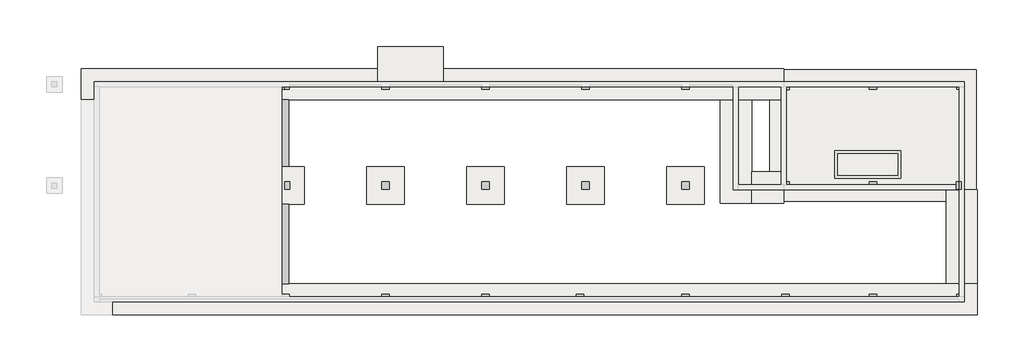
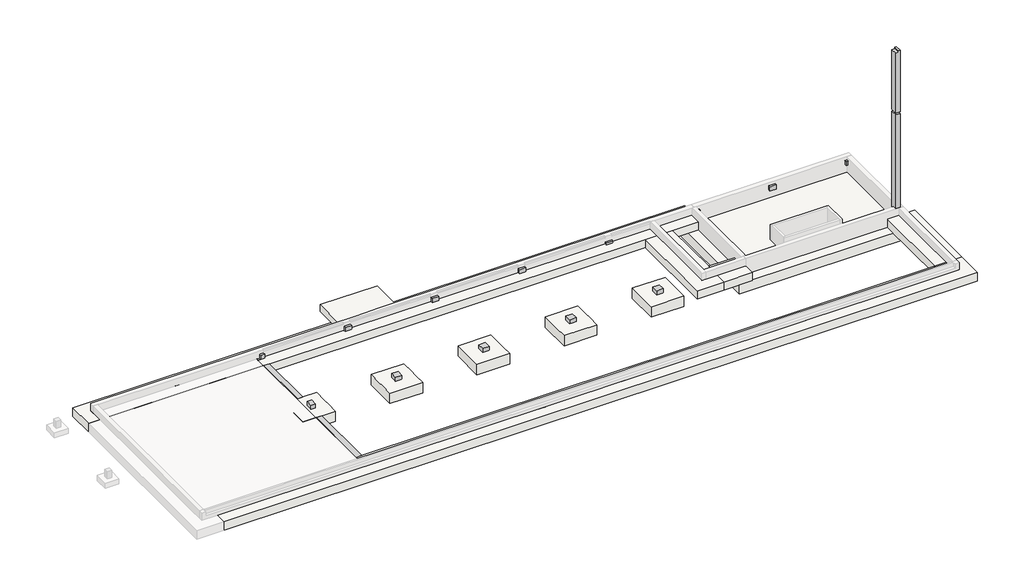
# Not in any storey, part 2 of 2: 25 columns, 8 beams, 8 slabs, 5 footings.
# Revit data of these elements (continued)
# Type "H_SF_AR_B01_MAT_Bitumen_MF2" (continued)
#   H_WM Code_3 = "A03AF036-00001 |  | M2 | Concrete Work | Superstructure Work | Form Work (1 time in use) | Flat Form | Dressed Lumber, Plywood or Steel Form(Wood Planks are not Allowed) incl. Chamfer |  |  |  | A03AF036-00001 Concrete Work Superstructure Work Form Work (1 time in use) Flat Form     Dressed Lumber, Plywood or Steel Form(Wood Planks are not Allowed) incl. Chamfer   |"
#   H_Rebar ratio = 0.12
#   Layers, outside or top first: 650 mm "00_Concrete_Reinf. Conc." (function 1)
# Type "Foundation Rectangular (Non-Pile) : H_SF_AR_S18_W2500xL2500xT1000_Bitumen_F1"
#   Type Comments = "CV-UG"
#   Type Mark = "F1"
#   H_Q'ty Cal Type Tag = "SC-Q1A"
#   H_WM Code_1 = "A03AD044-00001 |  | M | Concrete Work | Substructure Work | Isolation Joint (Separation Joint) | w/ Flexible Joint Filler, Sealant | THK=(  )mm |  | A03AD044-00001 Concrete Work Substructure Work Isolation Joint (Separation Joint)      w/ Flexible Joint Filler, Sealant   | THK=( 12 )mm"
#   H_WM Code_2 = "A03AD032-00022 |  | M3 | Concrete Work | Substructure Work | Structural Concrete | Cement Type-1 | 25MPa ≤ F'c (Cylinder Strength) < 30MPa |  |  |  |  | A03AD032-00022 Concrete Work Substructure Work Structural Concrete  Cement Type-1 25MPa ≤ F'c (Cylinder Strength) < 30MPa      |  F'c (Cylinder Strength) = 24MPa"
#   H_WM Code_3 = "A03AD037-00002 |  | TON | Concrete Work | Substructure Work | Rebar Work | Deformed Bar (Non-Coat.) | 400MPa<Fy≤470MPa |  |  |  |  | A03AD037-00002 Concrete Work Substructure Work Rebar Work Deformed Bar (Non-Coat.)  400MPa<Fy≤470MPa      | ASTM A615 GRADE 60 (Fy=420MPa)"
#   H_WM Code_4 = "A03AD035-00001 |  | M2 | Concrete Work | Substructure Work | Form Work (3 times in use) | Flat Form | Dressed Lumber, Plywood or Steel Form(Wood Planks are not Allowed) incl. Chamfer |  |  |  | A03AD035-00001 Concrete Work Substructure Work Form Work (3 times in use) Flat Form     Dressed Lumber, Plywood or Steel Form(Wood Planks are not Allowed) incl. Chamfer   |"
#   H_WM Code_5 = "A01ZZ003-00001 |  | M3 | Earth Work | - | Backfill | Re-use, Soil |  |  |  | Compaction=(  )% |  | A01ZZ003-00001 Earth Work - Backfill Re-use, Soil        | Compaction=( 95 )%"
#   H_WM Code_6 = "A01ZZ004-00001 |  | M3 | Earth Work | - | Disposal | Soil |  |  |  | Disposal Distance=Appx. (  )km from Site |  | A01ZZ004-00001 Earth Work - Disposal Soil        | Disposal Distance=Appx. (20 )km from Site"
#   H_WM Code_7 = "A03AH056-00001 |  | M2 | Concrete Work | Concrete Protective Coating (U/G) | Bitumen/Bituminous/Asphalt Coating |  |  | A03AH056-00001 Concrete Work Concrete Protective Coating (U/G) Bitumen/Bituminous/Asphalt Coating         |"
#   Top bar = "D25@300"
#   Description = "UG Shallow Foundation"
#   Bottom bar = "D20@300"
#   H_Rebar ratio = 0.12
#   Width = 3000 mm
#   Length = 3000 mm
#   Foundation Thickness = 1000 mm
#   Structural Material [instance default] = none
#   Assembly Code = ""
# Elements 1, 2 (IfcBeam, "RC Beam_Rectangular : H_SB_AR_S16_FG_B600xH800_FG2")
#   Comments = ""
#   hec_material3 = none
#   hec_material2 = none
#   hec_material1 = 00_Concrete_Reinf. Conc.
#   Structural Material = 00_Concrete_Reinf. Conc.
#   Phase Created = New Construction
#   Materials on its faces: "00_Concrete_Reinf. Conc."
# Elements 3, 4, 5 (IfcBeam, "RC Beam_Rectangular : H_SB_AR_S16_FG_B500xH700_FB1")
#   Comments = ""
#   hec_material3 = none
#   hec_material2 = none
#   hec_material1 = none
#   Structural Material = 00_Concrete_Reinf. Conc.
#   Phase Created = New Construction
#   Materials on its faces: "00_Concrete_Reinf. Conc."
# Elements 6, 7, 8 (IfcBeam, "RC Beam_Rectangular : H_SB_AR_S16_FG_B500xH700_FG1")
#   Comments = ""
#   hec_material3 = none
#   hec_material2 = none
#   hec_material1 = none
#   Structural Material = 00_Concrete_Reinf. Conc.
#   Phase Created = New Construction
#   Materials on its faces: "00_Concrete_Reinf. Conc."
# Element 9 (IfcColumn, "RC_Column_Rectangular : H_SC_AR_S15_UG_W600xL600_C2")
#   Comments = ""
#   H_Re Bar Ratio = 0.3
#   hec_material3 = none
#   hec_material2 = none
#   hec_material1 = none
#   Structural Material = 00_Concrete_Reinf. Conc.
#   Phase Created = New Construction
#   Materials on its faces: "00_Concrete_Reinf. Conc."
# Elements 10, 11, 12, 13, 14, 15, 16, 17, 18, 19, 20, 21, 22, 31, 32 (IfcColumn, "RC_Column_Rectangular : H_SC_AR_S15_UG_W600xL600_C2")
#   Comments = ""
#   hec_material3 = none
#   hec_material2 = none
#   hec_material1 = none
#   Structural Material = 00_Concrete_Reinf. Conc.
#   Phase Created = New Construction
#   Materials on its faces: "00_Concrete_Reinf. Conc."
# Elements 23, 24, 25, 26, 27, 28, 29, 30, 33 (IfcColumn, "RC_Column_Rectangular : H_SC_AR_S15_AG_W600xL600_C2")
#   Comments = ""
#   hec_material3 = none
#   hec_material2 = none
#   hec_material1 = none
#   Structural Material = 00_Concrete_Reinf. Conc.
#   Phase Created = New Construction
#   Materials on its faces: "00_Concrete_Reinf. Conc."
# Elements 34, 37, 38 (IfcFooting, "H_SF_AR_B01_Wall FDN_T800")
#   Comments = ""
#   Phase Created = New Construction
#   Materials on its faces: "00_Concrete_Reinf. Conc."
# Element 35 (IfcFooting, "H_SF_AR_B01_Wall FDN_T800")
#   Comments = ""
#   H_Re Bar Ratio = 0.3
#   Phase Created = New Construction
#   Materials on its faces: "00_Concrete_Reinf. Conc."
# Element 36 (IfcFooting, "H_SF_AR_B01_Wall FDN_T800")
#   Phase Created = New Construction
#   Materials on its faces: "00_Concrete_Reinf. Conc."
# Element 39 (IfcSlab, "H_SF_AR_B01_MAT_Bitumen_MF1")
#   Comments = ""
#   Height Offset From Level = 0 mm
#   built-in parameter 1001954 = 1
#   Phase Created = New Construction
#   Materials on its faces: "00_Concrete_Reinf. Conc."
# Element 40 (IfcSlab, "H_SF_AR_B01_MAT_Bitumen_MF2")
#   Comments = ""
#   Height Offset From Level = 1450 mm
#   built-in parameter 1001954 = 1
#   Phase Created = New Construction
#   Materials on its faces: "00_Concrete_Reinf. Conc."
# Elements 41, 42, 43, 44, 45, 46 (IfcSlab, "Foundation Rectangular (Non-Pile) : H_SF_AR_S18_W2500xL2500xT1000_Bitumen_F1")
#   Comments = ""
#   Structural Material = 00_Concrete_Reinf. Conc.
#   Phase Created = New Construction
#   Materials on its faces: "00_Concrete_Reinf. Conc."
# Materials
#   "00_Concrete_Reinf. Conc.": class "Concrete", colour RGB 176 176 176, transparency 0, Description = "Reinf. Conc.", Cost = 0, Image = Concrete.Cast-In-Place.Flat.Polished.Grey.jpg
